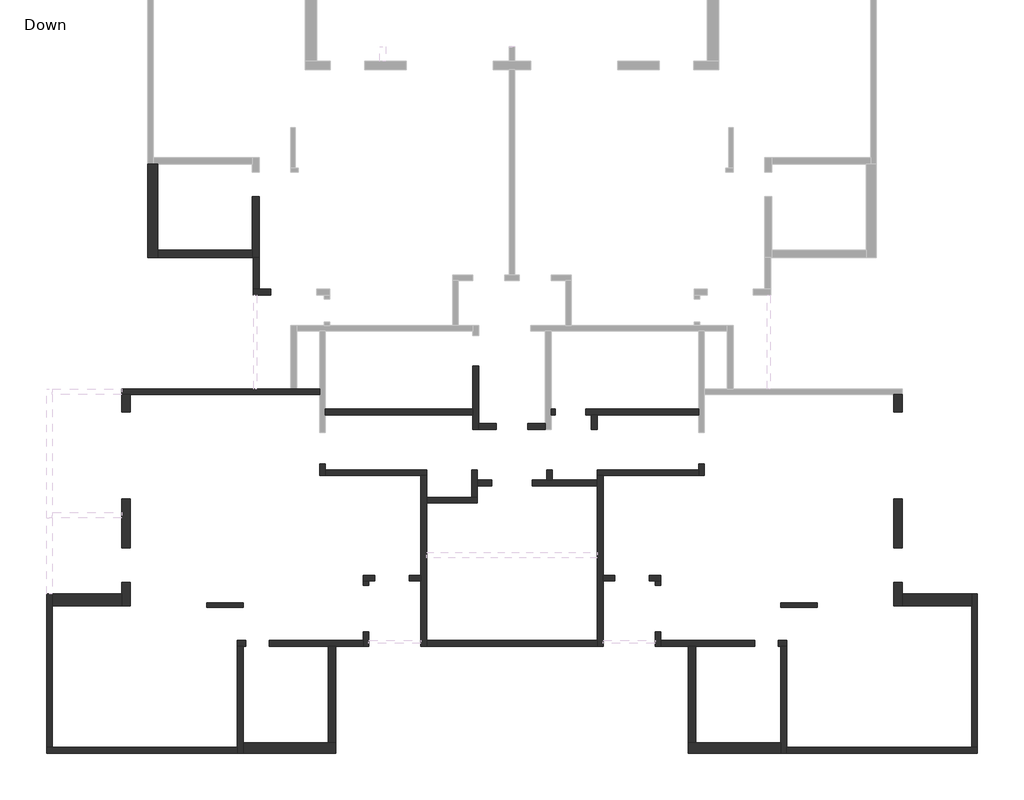
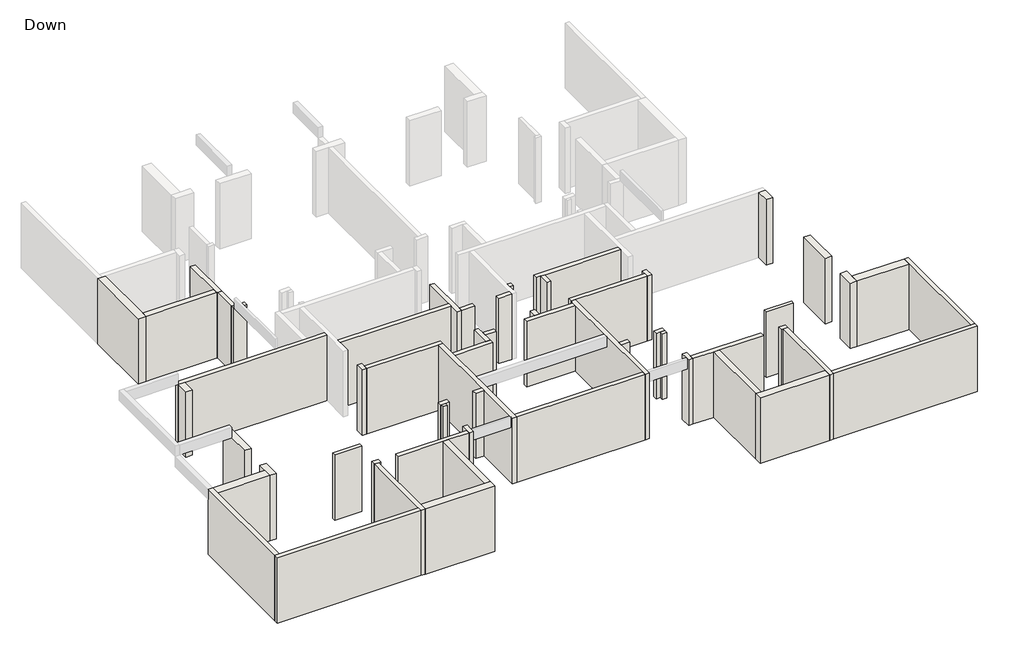
# One storey, part 1 of 2: 57 walls.
"""IFC4 building model written with IfcOpenShell, lengths in millimetres."""

import ifcopenshell
import ifcopenshell.guid

model = None  # the IFC model being written
_history = None  # IfcOwnerHistory: only IFC2X3 demands one
_inside = {}  # id of a spatial element -> (the spatial element, [elements in it])
_under = {}  # id of a project, library or spatial element -> (it, [spatial elements below it])
_declared = {}  # id of a project -> (the project, [libraries it declares])
_typed = {}  # id of a type object -> (the type object, [elements of that type])
_made_of = {}  # id of a material, layer set ... -> (it, [elements and type objects made of it])


def new_model(schema):
    """Start an empty IFC model of exactly this schema.

    Asked for "IFC4X3", IfcOpenShell would pick the latest addendum, in which some entities
    have other attributes; the version numbers below select the first issue.
    IFC2X3 requires an IfcOwnerHistory on every rooted entity: one is made here for all.
    """
    global model, _history
    if schema == "IFC4X3":
        model = ifcopenshell.file(schema_version=(4, 3, 0, 0))
    else:
        model = ifcopenshell.file(schema=schema)
    _inside.clear()
    _under.clear()
    _declared.clear()
    _typed.clear()
    _made_of.clear()
    _history = None
    if model.schema == "IFC2X3":
        org = make("IfcOrganization", Name="unknown")
        user = make(
            "IfcPersonAndOrganization",
            ThePerson=make("IfcPerson", FamilyName="unknown"),
            TheOrganization=org,
        )
        app = make(
            "IfcApplication",
            ApplicationDeveloper=org,
            Version="unknown",
            ApplicationFullName="unknown",
            ApplicationIdentifier="unknown",
        )
        _history = make(
            "IfcOwnerHistory",
            OwningUser=user,
            OwningApplication=app,
            ChangeAction="ADDED",
            CreationDate=0,
        )
    return model


def make(cls, **values):
    """One entity of the class cls with the attributes given. An attribute that is None is left unset."""
    return model.create_entity(
        cls, **{name: value for name, value in values.items() if value is not None}
    )


def rooted(cls, **values):
    """An entity with a GlobalId (a new one), such as an element, a storey or a relation."""
    return make(cls, GlobalId=ifcopenshell.guid.new(), OwnerHistory=_history, **values)


def si_unit(unit_type, name, prefix=None):
    """IfcSIUnit, for example si_unit("LENGTHUNIT", "METRE", prefix="MILLI")."""
    return make("IfcSIUnit", UnitType=unit_type, Prefix=prefix, Name=name)


def assignment(units):
    """IfcUnitAssignment: the units of a project."""
    return None if units is None else make("IfcUnitAssignment", Units=units)


def point(xyz):
    """IfcCartesianPoint."""
    return None if xyz is None else make("IfcCartesianPoint", Coordinates=xyz)


def direction(xyz):
    """IfcDirection."""
    return None if xyz is None else make("IfcDirection", DirectionRatios=xyz)


def frame(location, z_axis=None, x_axis=None):
    """IfcAxis2Placement3D, a coordinate frame: its origin and axes. An axis left out is left unset."""
    return make(
        "IfcAxis2Placement3D",
        Location=point(location),
        Axis=direction(z_axis),
        RefDirection=direction(x_axis),
    )


def origin():
    """The frame at (0, 0, 0) with its axes left unset."""
    return frame((0.0, 0.0, 0.0))


def origin_with_axes():
    """The frame at (0, 0, 0) with the z axis (0, 0, 1) and the x axis (1, 0, 0) written out."""
    return frame((0.0, 0.0, 0.0), z_axis=(0.0, 0.0, 1.0), x_axis=(1.0, 0.0, 0.0))


def place(relative_to, where):
    """IfcLocalPlacement: puts the frame where relative to a parent placement (None: the world)."""
    return make(
        "IfcLocalPlacement", PlacementRelTo=relative_to, RelativePlacement=where
    )


def context(
    kind, dimensions, precision=None, world=None, true_north=None, identifier=None
):
    """IfcGeometricRepresentationContext, for example the 3D "Model" context."""
    return make(
        "IfcGeometricRepresentationContext",
        ContextIdentifier=identifier,
        ContextType=kind,
        CoordinateSpaceDimension=dimensions,
        Precision=precision,
        WorldCoordinateSystem=world,
        TrueNorth=true_north,
    )


def project(units=None, contexts=None):
    """IfcProject with its units and contexts."""
    return rooted(
        "IfcProject",
        Name="project",
        RepresentationContexts=contexts,
        UnitsInContext=assignment(units),
    )


def spatial(cls, under=None, at=None, **own):
    """A site, building, storey or space (cls), placed at a placement, below another one or the project."""
    s = rooted(cls, ObjectPlacement=at, **own)
    if under is not None:
        _under.setdefault(under.id(), (under, []))[1].append(s)
    return s


def polyline(points):
    """IfcPolyline through the points."""
    return make("IfcPolyline", Points=[point(p) for p in points])


def outline(outer, holes=None, kind="AREA"):
    """IfcArbitraryClosedProfileDef: a profile drawn as a closed curve; with holes, ...WithVoids."""
    if holes is None:
        return make("IfcArbitraryClosedProfileDef", ProfileType=kind, OuterCurve=outer)
    return make(
        "IfcArbitraryProfileDefWithVoids",
        ProfileType=kind,
        OuterCurve=outer,
        InnerCurves=holes,
    )


def extrude(swept, where, along, depth):
    """IfcExtrudedAreaSolid: the profile swept, set in the frame where, extruded along a direction by depth."""
    return make(
        "IfcExtrudedAreaSolid",
        SweptArea=swept,
        Position=where,
        ExtrudedDirection=direction(along),
        Depth=depth,
    )


def faces_of(points, faces, orient=None, outer=None):
    """IfcFace entities. A face is a list of loops; a loop is a list of indices into points, from 0.

    orient and outer hold one flag for each loop. By default every Orientation is true, the
    first loop of a face is its IfcFaceOuterBound and the others are IfcFaceBound.
    """
    made = []
    for i, loops in enumerate(faces):
        bounds = []
        for j, loop in enumerate(loops):
            is_outer = j == 0 if outer is None else outer[i][j]
            bounds.append(
                make(
                    "IfcFaceOuterBound" if is_outer else "IfcFaceBound",
                    Bound=make("IfcPolyLoop", Polygon=[points[k] for k in loop]),
                    Orientation=True if orient is None else orient[i][j],
                )
            )
        made.append(make("IfcFace", Bounds=bounds))
    return made


def faceted_brep(points, faces, orient=None, outer=None, voids=None):
    """IfcFacetedBrep: a solid bounded by flat faces; with voids (closed shells), ...WithVoids."""
    shared = [point(p) for p in points]
    hull = make("IfcClosedShell", CfsFaces=faces_of(shared, faces, orient, outer))
    if voids is None:
        return make("IfcFacetedBrep", Outer=hull)
    return make(
        "IfcFacetedBrepWithVoids",
        Outer=hull,
        Voids=[
            make(cls, CfsFaces=faces_of(shared, fs, o, b)) for cls, fs, o, b in voids
        ],
    )


def shape(context_of_items, identifier, shape_type, items):
    """IfcShapeRepresentation: the items that make up one representation, for example the "Body"."""
    return make(
        "IfcShapeRepresentation",
        ContextOfItems=context_of_items,
        RepresentationIdentifier=identifier,
        RepresentationType=shape_type,
        Items=items,
    )


def made_of(thing, what):
    """Note that an element or type object is made of a material, layer set ...; save() writes the relation."""
    if what is not None:
        _made_of.setdefault(what.id(), (what, []))[1].append(thing)
    return thing


def element(
    cls,
    number,
    at=None,
    inside=None,
    cuts=None,
    type_object=None,
    material=None,
    context=None,
    identifier="Body",
    shape_type=None,
    held_by="IfcProductDefinitionShape",
    body=None,
    shapes=None,
    **own,
):
    """One element of the class cls, such as IfcWall. Its Tag is "e" and its number.

    at: its placement. inside: the storey or other place that contains it. cuts: it is an
    opening in that element (IfcRelVoidsElement). A single representation is given by context,
    identifier, shape_type and body (its items); several are given by shapes. held_by: the class
    of the entity that holds the representations. save() writes the other relations.
    """
    e = rooted(cls, Tag="e%d" % number, ObjectPlacement=at, **own)
    if body is not None:
        shapes = [shape(context, identifier, shape_type, body)]
    if shapes is not None:
        e.Representation = make(held_by, Representations=shapes)
    if inside is not None:
        _inside.setdefault(inside.id(), (inside, []))[1].append(e)
    if cuts is not None:
        rooted(
            "IfcRelVoidsElement", RelatingBuildingElement=cuts, RelatedOpeningElement=e
        )
    if type_object is not None:
        _typed.setdefault(type_object.id(), (type_object, []))[1].append(e)
    return made_of(e, material)


def aggregate(whole, parts):
    """IfcRelAggregates: a whole, such as a stair, and the parts it consists of."""
    return rooted("IfcRelAggregates", RelatingObject=whole, RelatedObjects=parts)


def save(model, path):
    """Write the relations noted so far, then the file.

    IfcRelAggregates (storeys below a building ...), IfcRelContainedInSpatialStructure (elements
    in a storey), IfcRelDefinesByType, IfcRelAssociatesMaterial and IfcRelDeclares: one each for
    every whole, place, type object, material and project.
    """
    for whole, parts in _under.values():
        aggregate(whole, parts)
    for where, things in _inside.values():
        rooted(
            "IfcRelContainedInSpatialStructure",
            RelatedElements=things,
            RelatingStructure=where,
        )
    for kind, things in _typed.values():
        rooted("IfcRelDefinesByType", RelatedObjects=things, RelatingType=kind)
    for what, things in _made_of.values():
        rooted("IfcRelAssociatesMaterial", RelatedObjects=things, RelatingMaterial=what)
    for by, libraries in _declared.values():
        rooted("IfcRelDeclares", RelatingContext=by, RelatedDefinitions=libraries)
    model.write(path)


model = new_model("IFC4")

# Units and contexts
model_context = context("Model", 3, world=origin())
ifc_project = project(units=[si_unit("LENGTHUNIT", "METRE", prefix="MILLI")], contexts=[model_context])

# Site, building, storey
site = spatial("IfcSite", under=ifc_project)
building = spatial("IfcBuilding", under=site)
storey = spatial("IfcBuildingStorey", under=building, Name="Down", Elevation=0.0)

# Walls
placement = place(None, origin())
element("IfcWall", 1, ObjectType="15", at=placement, inside=storey, context=model_context, shape_type="Brep", body=[
    faceted_brep([(-10394.9709719, -7272.1211235, 0.0), (-9144.0302381, -7272.1211235, 0.0), (-9144.0302381, -7272.1211235, 2980.0), (-9144.0302381, -7272.1211235, 3180.0), (-10394.9709719, -7272.1211235, 3180.0), (-10394.9709719, -7272.1211235, 2980.0), (-10394.9709719, -7122.1211235, 0.0), (-10394.9709719, -7122.1211235, 2980.0), (-10394.9709719, -7122.1211235, 3180.0), (-9144.0302381, -7122.1211235, 3180.0), (-9144.0302381, -7122.1211235, 2980.0), (-9144.0302381, -7122.1211235, 0.0)], [[[0, 1, 2, 3, 4, 5]], [[6, 7, 8, 9, 10, 11]], [[1, 0, 6, 11]], [[3, 2, 1, 11, 10, 9]], [[4, 3, 9, 8]], [[0, 5, 4, 8, 7, 6]]]),
])
element("IfcWall", 2, ObjectType="15", at=placement, inside=storey, context=model_context, shape_type="Brep", body=[
    faceted_brep([(10709.0741833, -7122.1211235, 0.0), (9458.1334495, -7122.1211235, 0.0), (9458.1334495, -7122.1211235, 2980.0), (9458.1334495, -7122.1211235, 3180.0), (10709.0741833, -7122.1211235, 3180.0), (10709.0741833, -7122.1211235, 2980.0), (10709.0741833, -7272.1211235, 0.0), (10709.0741833, -7272.1211235, 2980.0), (10709.0741833, -7272.1211235, 3180.0), (9458.1334495, -7272.1211235, 3180.0), (9458.1334495, -7272.1211235, 2980.0), (9458.1334495, -7272.1211235, 0.0)], [[[0, 1, 2, 3, 4, 5]], [[6, 7, 8, 9, 10, 11]], [[1, 0, 6, 11]], [[3, 2, 1, 11, 10, 9]], [[4, 3, 9, 8]], [[0, 5, 4, 8, 7, 6]]]),
])
element("IfcWall", 3, ObjectType="20", at=placement, inside=storey, context=model_context, shape_type="Brep", body=[
    faceted_brep([(-8793.7009813, 4828.7725736, 0.0), (-8793.7009813, 3729.1488671, 0.0), (-8793.7009813, 3729.1488671, 3180.0), (-8793.7009813, 4828.7725736, 3180.0), (-8593.7009813, 4828.7725736, 0.0), (-8593.7009813, 4828.7725736, 3180.0), (-8593.7009813, 3729.1488671, 3180.0), (-8593.7009813, 3729.1488671, 2980.0), (-8593.7009813, 3729.1488671, 0.0)], [[[0, 1, 2, 3]], [[4, 5, 6, 7, 8]], [[1, 0, 4, 8]], [[3, 2, 6, 5]], [[0, 3, 5, 4]], [[2, 1, 8, 7, 6]]]),
])
element("IfcWall", 4, ObjectType="20", at=placement, inside=storey, context=model_context, shape_type="Brep", body=[
    faceted_brep([(-8793.7009813, 3529.1488671, 0.0), (-8193.6539446, 3529.1488671, 0.0), (-8193.6539446, 3529.1488671, 2980.0), (-8193.6539446, 3529.1488671, 3180.0), (-8774.1337189, 3529.1488671, 3180.0), (-8793.7009813, 3529.1488671, 3180.0), (-8793.7009813, 3729.1488671, 0.0), (-8793.7009813, 3729.1488671, 3180.0), (-8593.7009813, 3729.1488671, 3180.0), (-8193.6539446, 3729.1488671, 3180.0), (-8193.6539446, 3729.1488671, 2980.0), (-8193.6539446, 3729.1488671, 0.0), (-8593.7009813, 3729.1488671, 0.0)], [[[0, 1, 2, 3, 4, 5]], [[6, 7, 8, 9, 10, 11, 12]], [[1, 0, 6, 12, 11]], [[3, 2, 1, 11, 10, 9]], [[5, 4, 3, 9, 8, 7]], [[0, 5, 7, 6]]]),
])
element("IfcWall", 5, ObjectType="20", at=placement, inside=storey, context=model_context, shape_type="Brep", body=[
    faceted_brep([(-1194.9239352, 1067.4837683, 0.0), (-1194.9239352, -421.6037199, 0.0), (-1194.9239352, -621.6037199, 0.0), (-1194.9239352, -1121.133353, 0.0), (-1194.9239352, -1121.133353, 2980.0), (-1194.9239352, -1121.133353, 3180.0), (-1194.9239352, -621.6037199, 3180.0), (-1194.9239352, -421.6037199, 3180.0), (-1194.9239352, 1067.4837683, 3180.0), (-1194.9239352, 1067.4837683, 2980.0), (-994.9239352, 1067.4837683, 0.0), (-994.9239352, 1067.4837683, 2980.0), (-994.9239352, 1067.4837683, 3180.0), (-994.9239352, -921.133353, 3180.0), (-994.9239352, -1121.133353, 3180.0), (-994.9239352, -1121.133353, 0.0), (-994.9239352, -921.133353, 0.0)], [[[0, 1, 2, 3, 4, 5, 6, 7, 8, 9]], [[10, 11, 12, 13, 14, 15, 16]], [[3, 2, 1, 0, 10, 16, 15]], [[8, 7, 6, 5, 14, 13, 12]], [[0, 9, 8, 12, 11, 10]], [[5, 4, 3, 15, 14]]]),
])
element("IfcWall", 6, ObjectType="20", at=placement, inside=storey, context=model_context, shape_type="Brep", body=[
    faceted_brep([(-994.9239352, -1121.133353, 0.0), (-393.7950547, -1121.133353, 0.0), (-393.7950547, -1121.133353, 2980.0), (-393.7950547, -1121.133353, 3180.0), (-994.9239352, -1121.133353, 3180.0), (-994.9239352, -921.133353, 0.0), (-994.9239352, -921.133353, 2980.0), (-994.9239352, -921.133353, 3180.0), (-393.7950547, -921.133353, 3180.0), (-393.7950547, -921.133353, 2980.0), (-393.7950547, -921.133353, 0.0)], [[[0, 1, 2, 3, 4]], [[5, 6, 7, 8, 9, 10]], [[1, 0, 5, 10]], [[3, 2, 1, 10, 9, 8]], [[4, 3, 8, 7]], [[0, 4, 7, 6, 5]]]),
])
element("IfcWall", 7, ObjectType="20", at=placement, inside=storey, context=model_context, shape_type="Brep", body=[
    faceted_brep([(-1194.9239352, -421.6037199, 0.0), (-6295.0180086, -421.6037199, 0.0), (-6295.0180086, -421.6037199, 3180.0), (-1194.9239352, -421.6037199, 3180.0), (-1194.9239352, -621.6037199, 0.0), (-1194.9239352, -621.6037199, 2980.0), (-1194.9239352, -621.6037199, 3180.0), (-6295.0180086, -621.6037199, 3180.0), (-6295.0180086, -621.6037199, 2980.0), (-6295.0180086, -621.6037199, 0.0)], [[[0, 1, 2, 3]], [[4, 5, 6, 7, 8, 9]], [[1, 0, 4, 9]], [[3, 2, 7, 6]], [[0, 3, 6, 5, 4]], [[2, 1, 9, 8, 7]]]),
])
element("IfcWall", 8, ObjectType="20", at=placement, inside=storey, context=model_context, shape_type="Brep", body=[
    faceted_brep([(-6495.0180086, 279.007757, 0.0), (-7293.0424677, 279.007757, 0.0), (-7493.0424677, 279.007757, 0.0), (-13343.4657979, 279.007757, 0.0), (-13343.4657979, 279.007757, 2980.0), (-13343.4657979, 279.007757, 3180.0), (-8774.1337189, 279.007757, 3180.0), (-7493.0424677, 279.007757, 3180.0), (-7293.0424677, 279.007757, 3180.0), (-6495.0180086, 279.007757, 3180.0), (-6495.0180086, 79.007757, 0.0), (-6495.0180086, 79.007757, 2980.0), (-6495.0180086, 79.007757, 3180.0), (-13042.9013576, 79.007757, 3180.0), (-13342.9013576, 79.007757, 3180.0), (-13343.4657979, 79.007757, 3180.0), (-13343.4657979, 79.007757, 2980.0), (-13343.4657979, 79.007757, 0.0), (-13342.9013576, 79.007757, 0.0), (-13042.9013576, 79.007757, 0.0)], [[[0, 1, 2, 3, 4, 5, 6, 7, 8, 9]], [[10, 11, 12, 13, 14, 15, 16, 17, 18, 19]], [[3, 2, 1, 0, 10, 19, 18, 17]], [[5, 4, 3, 17, 16, 15]], [[9, 8, 7, 6, 5, 15, 14, 13, 12]], [[0, 9, 12, 11, 10]]]),
])
element("IfcWall", 9, ObjectType="20", at=placement, inside=storey, context=model_context, shape_type="Brep", body=[
    faceted_brep([(-6493.9832015, -2321.2744631, 0.0), (-6493.9832015, -2721.3214998, 0.0), (-6493.9832015, -2721.3214998, 2980.0), (-6493.9832015, -2721.3214998, 3180.0), (-6493.9832015, -2321.2744631, 3180.0), (-6493.9832015, -2321.2744631, 2980.0), (-6293.9832015, -2321.2744631, 0.0), (-6293.9832015, -2321.2744631, 2980.0), (-6293.9832015, -2321.2744631, 3180.0), (-6293.9832015, -2521.3214998, 3180.0), (-6293.9832015, -2721.3214998, 3180.0), (-6293.9832015, -2721.3214998, 0.0), (-6293.9832015, -2521.3214998, 0.0), (-6295.0180086, -2321.2744631, 3180.0)], [[[0, 1, 2, 3, 4, 5]], [[6, 7, 8, 9, 10, 11, 12]], [[1, 0, 6, 12, 11]], [[4, 3, 10, 9, 8, 13]], [[0, 5, 4, 13, 8, 7, 6]], [[3, 2, 1, 11, 10]]]),
])
element("IfcWall", 10, ObjectType="20", at=placement, inside=storey, context=model_context, shape_type="Brep", body=[
    faceted_brep([(-6293.9832015, -2721.3214998, 0.0), (-2993.9832015, -2721.3214998, 0.0), (-2793.9832015, -2721.3214998, 0.0), (-2793.9832015, -2721.3214998, 3180.0), (-2993.9832015, -2721.3214998, 3180.0), (-6293.9832015, -2721.3214998, 3180.0), (-6293.9832015, -2521.3214998, 0.0), (-6293.9832015, -2521.3214998, 2980.0), (-6293.9832015, -2521.3214998, 3180.0), (-2793.9832015, -2521.3214998, 3180.0), (-2793.9832015, -2521.3214998, 2980.0), (-2793.9832015, -2521.3214998, 0.0)], [[[0, 1, 2, 3, 4, 5]], [[6, 7, 8, 9, 10, 11]], [[2, 1, 0, 6, 11]], [[5, 4, 3, 9, 8]], [[0, 5, 8, 7, 6]], [[3, 2, 11, 10, 9]]]),
])
element("IfcWall", 11, ObjectType="20", at=placement, inside=storey, context=model_context, shape_type="Brep", body=[
    faceted_brep([(-2993.9832015, -2721.3214998, 0.0), (-2993.9832015, -6171.4626098, 0.0), (-2993.9832015, -6371.4626098, 0.0), (-2993.9832015, -8622.5444537, 0.0), (-2993.9832015, -8622.5444537, 3180.0), (-2993.9832015, -8420.9452063, 3180.0), (-2993.9832015, -6371.4626098, 3180.0), (-2993.9832015, -6171.4626098, 3180.0), (-2993.9832015, -2721.3214998, 3180.0), (-2993.9832015, -2721.3214998, 2980.0), (-2793.9832015, -2721.3214998, 0.0), (-2793.9832015, -2721.3214998, 3180.0), (-2793.9832015, -3471.6977933, 3180.0), (-2793.9832015, -3671.6977933, 3180.0), (-2793.9832015, -5372.4503803, 3180.0), (-2793.9832015, -8422.5444537, 3180.0), (-2793.9832015, -8622.5444537, 3180.0), (-2793.9832015, -8622.5444537, 0.0), (-2793.9832015, -8422.5444537, 0.0), (-2793.9832015, -3671.6977933, 0.0), (-2793.9832015, -3471.6977933, 0.0)], [[[0, 1, 2, 3, 4, 5, 6, 7, 8, 9]], [[10, 11, 12, 13, 14, 15, 16, 17, 18, 19, 20]], [[3, 2, 1, 0, 10, 20, 19, 18, 17]], [[8, 7, 6, 5, 4, 16, 15, 14, 13, 12, 11]], [[0, 9, 8, 11, 10]], [[4, 3, 17, 16]]]),
])
element("IfcWall", 12, ObjectType="20", at=placement, inside=storey, context=model_context, shape_type="Brep", body=[
    faceted_brep([(-2993.9832015, -6171.4626098, 0.0), (-3395.2061554, -6171.4626098, 0.0), (-3395.2061554, -6171.4626098, 2980.0), (-3395.2061554, -6171.4626098, 3180.0), (-2993.9832015, -6171.4626098, 3180.0), (-2993.9832015, -6171.4626098, 2980.0), (-2993.9832015, -6371.4626098, 0.0), (-2993.9832015, -6371.4626098, 2980.0), (-2993.9832015, -6371.4626098, 3180.0), (-3395.2061554, -6371.4626098, 3180.0), (-3395.2061554, -6371.4626098, 2980.0), (-3395.2061554, -6371.4626098, 0.0)], [[[0, 1, 2, 3, 4, 5]], [[6, 7, 8, 9, 10, 11]], [[1, 0, 6, 11]], [[3, 2, 1, 11, 10, 9]], [[4, 3, 9, 8]], [[0, 5, 4, 8, 7, 6]]]),
])
element("IfcWall", 13, ObjectType="20", at=placement, inside=storey, context=model_context, shape_type="Brep", body=[
    faceted_brep([(-4595.3472654, -6171.4626098, 0.0), (-4993.2776511, -6171.4626098, 0.0), (-4993.2776511, -6171.4626098, 2980.0), (-4993.2776511, -6171.4626098, 3180.0), (-4595.3472654, -6171.4626098, 3180.0), (-4595.3472654, -6171.4626098, 2980.0), (-4595.3472654, -6371.4626098, 0.0), (-4595.3472654, -6371.4626098, 2980.0), (-4595.3472654, -6371.4626098, 3180.0), (-4793.2776511, -6371.4626098, 3180.0), (-4993.2776511, -6371.4626098, 3180.0), (-4993.2776511, -6371.4626098, 0.0), (-4793.2776511, -6371.4626098, 0.0)], [[[0, 1, 2, 3, 4, 5]], [[6, 7, 8, 9, 10, 11, 12]], [[1, 0, 6, 12, 11]], [[4, 3, 10, 9, 8]], [[0, 5, 4, 8, 7, 6]], [[3, 2, 1, 11, 10]]]),
])
element("IfcWall", 14, ObjectType="20", at=placement, inside=storey, context=model_context, shape_type="Brep", body=[
    faceted_brep([(-4993.2776511, -6371.4626098, 0.0), (-4993.2776511, -6522.8266738, 0.0), (-4993.2776511, -6522.8266738, 2980.0), (-4993.2776511, -6522.8266738, 3180.0), (-4993.2776511, -6371.4626098, 3180.0), (-4793.2776511, -6371.4626098, 0.0), (-4793.2776511, -6371.4626098, 2980.0), (-4793.2776511, -6371.4626098, 3180.0), (-4793.2776511, -6522.8266738, 3180.0), (-4793.2776511, -6522.8266738, 2980.0), (-4793.2776511, -6522.8266738, 0.0)], [[[0, 1, 2, 3, 4]], [[5, 6, 7, 8, 9, 10]], [[1, 0, 5, 10]], [[3, 2, 1, 10, 9, 8]], [[4, 3, 8, 7]], [[0, 4, 7, 6, 5]]]),
])
element("IfcWall", 15, ObjectType="20", at=placement, inside=storey, context=model_context, shape_type="Brep", body=[
    faceted_brep([(-4993.2776511, -8120.8981696, 0.0), (-4993.2776511, -8422.5444537, 0.0), (-4993.2776511, -8622.5444537, 0.0), (-4993.2776511, -8622.5444537, 3180.0), (-4993.2776511, -8422.5444537, 3180.0), (-4993.2776511, -8120.8981696, 3180.0), (-4993.2776511, -8120.8981696, 2980.0), (-4793.2776511, -8120.8981696, 0.0), (-4793.2776511, -8120.8981696, 2980.0), (-4793.2776511, -8120.8981696, 3180.0), (-4793.2776511, -8420.9452063, 3180.0), (-4793.2776511, -8622.5444537, 3180.0), (-4793.2776511, -8622.5444537, 0.0)], [[[0, 1, 2, 3, 4, 5, 6]], [[7, 8, 9, 10, 11, 12]], [[2, 1, 0, 7, 12]], [[5, 4, 3, 11, 10, 9]], [[0, 6, 5, 9, 8, 7]], [[3, 2, 12, 11]]]),
])
element("IfcWall", 16, ObjectType="20", at=placement, inside=storey, context=model_context, shape_type="Brep", body=[
    faceted_brep([(-4993.2776511, -8422.5444537, 0.0), (-8238.1036154, -8422.5444537, 0.0), (-8238.1036154, -8422.5444537, 2980.0), (-8238.1036154, -8422.5444537, 3180.0), (-4993.2776511, -8422.5444537, 3180.0), (-4993.2776511, -8422.5444537, 2980.0), (-4993.2776511, -8622.5444537, 0.0), (-4993.2776511, -8622.5444537, 3180.0), (-5943.7809437, -8622.5444537, 3180.0), (-6193.7809437, -8622.5444537, 3180.0), (-8238.1036154, -8622.5444537, 3180.0), (-8238.1036154, -8622.5444537, 2980.0), (-8238.1036154, -8622.5444537, 0.0), (-6193.7809437, -8622.5444537, 0.0), (-5943.7809437, -8622.5444537, 0.0)], [[[0, 1, 2, 3, 4, 5]], [[6, 7, 8, 9, 10, 11, 12, 13, 14]], [[1, 0, 6, 14, 13, 12]], [[3, 2, 1, 12, 11, 10]], [[4, 3, 10, 9, 8, 7]], [[0, 5, 4, 7, 6]]]),
])
element("IfcWall", 17, ObjectType="20", at=placement, inside=storey, context=model_context, shape_type="Brep", body=[
    faceted_brep([(-9048.7809437, -8422.5444537, 0.0), (-9343.7809437, -8422.5444537, 0.0), (-9343.7809437, -8422.5444537, 2980.0), (-9343.7809437, -8422.5444537, 3180.0), (-9048.7809437, -8422.5444537, 3180.0), (-9048.7809437, -8422.5444537, 2980.0), (-9048.7809437, -8622.5444537, 0.0), (-9048.7809437, -8622.5444537, 2980.0), (-9048.7809437, -8622.5444537, 3180.0), (-9143.7809437, -8622.5444537, 3180.0), (-9343.7809437, -8622.5444537, 3180.0), (-9343.7809437, -8622.5444537, 0.0), (-9143.7809437, -8622.5444537, 0.0)], [[[0, 1, 2, 3, 4, 5]], [[6, 7, 8, 9, 10, 11, 12]], [[1, 0, 6, 12, 11]], [[4, 3, 10, 9, 8]], [[0, 5, 4, 8, 7, 6]], [[3, 2, 1, 11, 10]]]),
])
element("IfcWall", 18, ObjectType="20", at=placement, inside=storey, context=model_context, shape_type="Brep", body=[
    faceted_brep([(-9343.7809437, -8622.5444537, 0.0), (-9343.7809437, -12122.4503803, 0.0), (-9343.7809437, -12322.4503803, 0.0), (-9343.7809437, -12322.4503803, 3180.0), (-9343.7809437, -12122.4503803, 3180.0), (-9343.7809437, -8622.5444537, 3180.0), (-9143.7809437, -8622.5444537, 0.0), (-9143.7809437, -8622.5444537, 2980.0), (-9143.7809437, -8622.5444537, 3180.0), (-9143.7809437, -11972.4503803, 3180.0), (-9143.7809437, -12322.4503803, 3180.0), (-9143.7809437, -12322.4503803, 0.0), (-9143.7809437, -11972.4503803, 0.0)], [[[0, 1, 2, 3, 4, 5]], [[6, 7, 8, 9, 10, 11, 12]], [[2, 1, 0, 6, 12, 11]], [[5, 4, 3, 10, 9, 8]], [[0, 5, 8, 7, 6]], [[3, 2, 11, 10]]]),
])
element("IfcWall", 19, ObjectType="20", at=placement, inside=storey, context=model_context, shape_type="Brep", body=[
    faceted_brep([(-9343.7809437, -12122.4503803, 0.0), (-15742.7132109, -12122.4503803, 0.0), (-15942.7132109, -12122.4503803, 0.0), (-15942.7132109, -12122.4503803, 3180.0), (-15742.7132109, -12122.4503803, 3180.0), (-9343.7809437, -12122.4503803, 3180.0), (-9343.7809437, -12122.4503803, 2980.0), (-9343.7809437, -12322.4503803, 0.0), (-9343.7809437, -12322.4503803, 3180.0), (-15942.7132109, -12322.4503803, 3180.0), (-15942.7132109, -12322.4503803, 0.0)], [[[0, 1, 2, 3, 4, 5, 6]], [[7, 8, 9, 10]], [[2, 1, 0, 7, 10]], [[5, 4, 3, 9, 8]], [[3, 2, 10, 9]], [[0, 6, 5, 8, 7]]]),
])
element("IfcWall", 20, ObjectType="20", at=placement, inside=storey, context=model_context, shape_type="Brep", body=[
    faceted_brep([(-15742.7132109, -12122.4503803, 0.0), (-15742.7132109, -7221.2744631, 0.0), (-15742.7132109, -6821.2744631, 0.0), (-15742.7132109, -6821.2744631, 2680.0), (-15742.7132109, -6821.2744631, 3180.0), (-15742.7132109, -7221.2744631, 3180.0), (-15742.7132109, -12122.4503803, 3180.0), (-15742.7132109, -12122.4503803, 2980.0), (-15942.7132109, -12122.4503803, 0.0), (-15942.7132109, -12122.4503803, 3180.0), (-15942.7132109, -6821.2744631, 3180.0), (-15942.7132109, -6821.2744631, 2680.0), (-15942.7132109, -6821.2744631, 0.0)], [[[0, 1, 2, 3, 4, 5, 6, 7]], [[8, 9, 10, 11, 12]], [[2, 1, 0, 8, 12]], [[6, 5, 4, 10, 9]], [[0, 7, 6, 9, 8]], [[4, 3, 2, 12, 11, 10]]]),
])
element("IfcWall", 21, ObjectType="20", at=placement, inside=storey, context=model_context, shape_type="Brep", body=[
    faceted_brep([(1309.0271466, -921.133353, 0.0), (707.8982661, -921.133353, 0.0), (707.8982661, -921.133353, 2980.0), (707.8982661, -921.133353, 3180.0), (1309.0271466, -921.133353, 3180.0), (1309.0271466, -921.133353, 2980.0), (1309.0271466, -1121.133353, 0.0), (1309.0271466, -1121.133353, 3180.0), (707.8982661, -1121.133353, 3180.0), (707.8982661, -1121.133353, 2980.0), (707.8982661, -1121.133353, 0.0)], [[[0, 1, 2, 3, 4, 5]], [[6, 7, 8, 9, 10]], [[1, 0, 6, 10]], [[3, 2, 1, 10, 9, 8]], [[4, 3, 8, 7]], [[0, 5, 4, 7, 6]]]),
])
element("IfcWall", 22, ObjectType="20", at=placement, inside=storey, context=model_context, shape_type="Brep", body=[
    faceted_brep([(2709.12122, -621.6037199, 0.0), (2906.0638352, -621.6037199, 0.0), (3106.0638352, -621.6037199, 0.0), (6609.12122, -621.6037199, 0.0), (6609.12122, -621.6037199, 2980.0), (6609.12122, -621.6037199, 3180.0), (3106.0638352, -621.6037199, 3180.0), (2906.0638352, -621.6037199, 3180.0), (2709.12122, -621.6037199, 3180.0), (2709.12122, -621.6037199, 2980.0), (2709.12122, -421.6037199, 0.0), (2709.12122, -421.6037199, 2980.0), (2709.12122, -421.6037199, 3180.0), (6609.12122, -421.6037199, 3180.0), (6609.12122, -421.6037199, 0.0)], [[[0, 1, 2, 3, 4, 5, 6, 7, 8, 9]], [[10, 11, 12, 13, 14]], [[3, 2, 1, 0, 10, 14]], [[8, 7, 6, 5, 13, 12]], [[0, 9, 8, 12, 11, 10]], [[5, 4, 3, 14, 13]]]),
])
element("IfcWall", 23, ObjectType="20", at=placement, inside=storey, context=model_context, shape_type="Brep", body=[
    faceted_brep([(6608.0864128, -2321.2744631, 0.0), (6608.0864128, -2521.3214998, 0.0), (6608.0864128, -2721.3214998, 0.0), (6608.0864128, -2721.3214998, 3180.0), (6608.0864128, -2521.3214998, 3180.0), (6608.0864128, -2321.2744631, 3180.0), (6608.0864128, -2321.2744631, 2980.0), (6808.0864128, -2321.2744631, 0.0), (6808.0864128, -2321.2744631, 2980.0), (6808.0864128, -2321.2744631, 3180.0), (6808.0864128, -2721.3214998, 3180.0), (6808.0864128, -2721.3214998, 2980.0), (6808.0864128, -2721.3214998, 0.0), (6609.12122, -2321.2744631, 3180.0)], [[[0, 1, 2, 3, 4, 5, 6]], [[7, 8, 9, 10, 11, 12]], [[2, 1, 0, 7, 12]], [[5, 4, 3, 10, 9, 13]], [[0, 6, 5, 13, 9, 8, 7]], [[3, 2, 12, 11, 10]]]),
])
element("IfcWall", 24, ObjectType="20", at=placement, inside=storey, context=model_context, shape_type="Brep", body=[
    faceted_brep([(6608.0864128, -2521.3214998, 0.0), (3108.0864128, -2521.3214998, 0.0), (3108.0864128, -2521.3214998, 2980.0), (3108.0864128, -2521.3214998, 3180.0), (6608.0864128, -2521.3214998, 3180.0), (6608.0864128, -2521.3214998, 2980.0), (6608.0864128, -2721.3214998, 0.0), (6608.0864128, -2721.3214998, 3180.0), (3308.0864128, -2721.3214998, 3180.0), (3108.0864128, -2721.3214998, 3180.0), (3108.0864128, -2721.3214998, 0.0), (3308.0864128, -2721.3214998, 0.0)], [[[0, 1, 2, 3, 4, 5]], [[6, 7, 8, 9, 10, 11]], [[1, 0, 6, 11, 10]], [[4, 3, 9, 8, 7]], [[0, 5, 4, 7, 6]], [[3, 2, 1, 10, 9]]]),
])
element("IfcWall", 25, ObjectType="20", at=placement, inside=storey, context=model_context, shape_type="Brep", body=[
    faceted_brep([(3108.0864128, -2721.3214998, 0.0), (3108.0864128, -2872.6855637, 0.0), (3108.0864128, -3072.6855637, 0.0), (3108.0864128, -8422.5444537, 0.0), (3108.0864128, -8622.5444537, 0.0), (3108.0864128, -8622.5444537, 3180.0), (3108.0864128, -8422.5444537, 3180.0), (3108.0864128, -5372.4503803, 3180.0), (3108.0864128, -3072.6855637, 3180.0), (3108.0864128, -2872.6855637, 3180.0), (3108.0864128, -2721.3214998, 3180.0), (3308.0864128, -2721.3214998, 0.0), (3308.0864128, -2721.3214998, 2980.0), (3308.0864128, -2721.3214998, 3180.0), (3308.0864128, -6171.4626098, 3180.0), (3308.0864128, -6371.4626098, 3180.0), (3308.0864128, -8420.9495778, 3180.0), (3308.0864128, -8622.5444537, 3180.0), (3308.0864128, -8622.5444537, 0.0), (3308.0864128, -6371.4626098, 0.0), (3308.0864128, -6171.4626098, 0.0)], [[[0, 1, 2, 3, 4, 5, 6, 7, 8, 9, 10]], [[11, 12, 13, 14, 15, 16, 17, 18, 19, 20]], [[4, 3, 2, 1, 0, 11, 20, 19, 18]], [[10, 9, 8, 7, 6, 5, 17, 16, 15, 14, 13]], [[0, 10, 13, 12, 11]], [[5, 4, 18, 17]]]),
])
element("IfcWall", 26, ObjectType="20", at=placement, inside=storey, context=model_context, shape_type="Brep", body=[
    faceted_brep([(3308.0864128, -6371.4626098, 0.0), (3709.3093668, -6371.4626098, 0.0), (3709.3093668, -6371.4626098, 2980.0), (3709.3093668, -6371.4626098, 3180.0), (3308.0864128, -6371.4626098, 3180.0), (3308.0864128, -6371.4626098, 2980.0), (3308.0864128, -6171.4626098, 0.0), (3308.0864128, -6171.4626098, 2980.0), (3308.0864128, -6171.4626098, 3180.0), (3709.3093668, -6171.4626098, 3180.0), (3709.3093668, -6171.4626098, 2980.0), (3709.3093668, -6171.4626098, 0.0)], [[[0, 1, 2, 3, 4, 5]], [[6, 7, 8, 9, 10, 11]], [[1, 0, 6, 11]], [[3, 2, 1, 11, 10, 9]], [[4, 3, 9, 8]], [[0, 5, 4, 8, 7, 6]]]),
])
element("IfcWall", 27, ObjectType="20", at=placement, inside=storey, context=model_context, shape_type="Brep", body=[
    faceted_brep([(4909.4504768, -6371.4626098, 0.0), (5107.3808625, -6371.4626098, 0.0), (5307.3808625, -6371.4626098, 0.0), (5307.3808625, -6371.4626098, 3180.0), (5107.3808625, -6371.4626098, 3180.0), (4909.4504768, -6371.4626098, 3180.0), (4909.4504768, -6371.4626098, 2980.0), (4909.4504768, -6171.4626098, 0.0), (4909.4504768, -6171.4626098, 2980.0), (4909.4504768, -6171.4626098, 3180.0), (5307.3808625, -6171.4626098, 3180.0), (5307.3808625, -6171.4626098, 2980.0), (5307.3808625, -6171.4626098, 0.0)], [[[0, 1, 2, 3, 4, 5, 6]], [[7, 8, 9, 10, 11, 12]], [[2, 1, 0, 7, 12]], [[5, 4, 3, 10, 9]], [[0, 6, 5, 9, 8, 7]], [[3, 2, 12, 11, 10]]]),
])
element("IfcWall", 28, ObjectType="20", at=placement, inside=storey, context=model_context, shape_type="Brep", body=[
    faceted_brep([(5107.3808625, -6371.4626098, 0.0), (5107.3808625, -6522.8266738, 0.0), (5107.3808625, -6522.8266738, 2980.0), (5107.3808625, -6522.8266738, 3180.0), (5107.3808625, -6371.4626098, 3180.0), (5107.3808625, -6371.4626098, 2980.0), (5307.3808625, -6371.4626098, 0.0), (5307.3808625, -6371.4626098, 3180.0), (5307.3808625, -6522.8266738, 3180.0), (5307.3808625, -6522.8266738, 2980.0), (5307.3808625, -6522.8266738, 0.0)], [[[0, 1, 2, 3, 4, 5]], [[6, 7, 8, 9, 10]], [[1, 0, 6, 10]], [[3, 2, 1, 10, 9, 8]], [[4, 3, 8, 7]], [[0, 5, 4, 7, 6]]]),
])
element("IfcWall", 29, ObjectType="20", at=placement, inside=storey, context=model_context, shape_type="Brep", body=[
    faceted_brep([(5107.3808625, -8120.8981696, 0.0), (5107.3808625, -8622.5444537, 0.0), (5107.3808625, -8622.5444537, 3180.0), (5107.3808625, -8420.9495778, 3180.0), (5107.3808625, -8120.8981696, 3180.0), (5107.3808625, -8120.8981696, 2980.0), (5307.3808625, -8120.8981696, 0.0), (5307.3808625, -8120.8981696, 2980.0), (5307.3808625, -8120.8981696, 3180.0), (5307.3808625, -8422.5444537, 3180.0), (5307.3808625, -8622.5444537, 3180.0), (5307.3808625, -8622.5444537, 0.0), (5307.3808625, -8422.5444537, 0.0)], [[[0, 1, 2, 3, 4, 5]], [[6, 7, 8, 9, 10, 11, 12]], [[1, 0, 6, 12, 11]], [[4, 3, 2, 10, 9, 8]], [[0, 5, 4, 8, 7, 6]], [[2, 1, 11, 10]]]),
])
element("IfcWall", 30, ObjectType="20", at=placement, inside=storey, context=model_context, shape_type="Brep", body=[
    faceted_brep([(5307.3808625, -8622.5444537, 0.0), (6257.8841551, -8622.5444537, 0.0), (6507.8841551, -8622.5444537, 0.0), (8552.2068268, -8622.5444537, 0.0), (8552.2068268, -8622.5444537, 2980.0), (8552.2068268, -8622.5444537, 3180.0), (6507.8841551, -8622.5444537, 3180.0), (6257.8841551, -8622.5444537, 3180.0), (5307.3808625, -8622.5444537, 3180.0), (5307.3808625, -8422.5444537, 0.0), (5307.3808625, -8422.5444537, 2980.0), (5307.3808625, -8422.5444537, 3180.0), (8552.2068268, -8422.5444537, 3180.0), (8552.2068268, -8422.5444537, 2980.0), (8552.2068268, -8422.5444537, 0.0)], [[[0, 1, 2, 3, 4, 5, 6, 7, 8]], [[9, 10, 11, 12, 13, 14]], [[3, 2, 1, 0, 9, 14]], [[5, 4, 3, 14, 13, 12]], [[8, 7, 6, 5, 12, 11]], [[0, 8, 11, 10, 9]]]),
])
element("IfcWall", 31, ObjectType="20", at=placement, inside=storey, context=model_context, shape_type="Brep", body=[
    faceted_brep([(9362.8841551, -8622.5444537, 0.0), (9457.8841551, -8622.5444537, 0.0), (9657.8841551, -8622.5444537, 0.0), (9657.8841551, -8622.5444537, 3180.0), (9457.8841551, -8622.5444537, 3180.0), (9362.8841551, -8622.5444537, 3180.0), (9362.8841551, -8622.5444537, 2980.0), (9362.8841551, -8422.5444537, 0.0), (9362.8841551, -8422.5444537, 2980.0), (9362.8841551, -8422.5444537, 3180.0), (9657.8841551, -8422.5444537, 3180.0), (9657.8841551, -8422.5444537, 2980.0), (9657.8841551, -8422.5444537, 0.0)], [[[0, 1, 2, 3, 4, 5, 6]], [[7, 8, 9, 10, 11, 12]], [[2, 1, 0, 7, 12]], [[5, 4, 3, 10, 9]], [[0, 6, 5, 9, 8, 7]], [[3, 2, 12, 11, 10]]]),
])
element("IfcWall", 32, ObjectType="20", at=placement, inside=storey, context=model_context, shape_type="Brep", body=[
    faceted_brep([(9457.8841551, -8622.5444537, 0.0), (9457.8841551, -11972.4503803, 0.0), (9457.8841551, -12322.4503803, 0.0), (9457.8841551, -12322.4503803, 3180.0), (9457.8841551, -11972.4503803, 3180.0), (9457.8841551, -8622.5444537, 3180.0), (9457.8841551, -8622.5444537, 2980.0), (9657.8841551, -8622.5444537, 0.0), (9657.8841551, -8622.5444537, 3180.0), (9657.8841551, -12122.4503803, 3180.0), (9657.8841551, -12322.4503803, 3180.0), (9657.8841551, -12322.4503803, 0.0), (9657.8841551, -12122.4503803, 0.0)], [[[0, 1, 2, 3, 4, 5, 6]], [[7, 8, 9, 10, 11, 12]], [[2, 1, 0, 7, 12, 11]], [[5, 4, 3, 10, 9, 8]], [[0, 6, 5, 8, 7]], [[3, 2, 11, 10]]]),
])
element("IfcWall", 33, ObjectType="20", at=placement, inside=storey, context=model_context, shape_type="Brep", body=[
    faceted_brep([(9657.8841551, -12322.4503803, 0.0), (16256.8164223, -12322.4503803, 0.0), (16256.8164223, -12322.4503803, 3180.0), (9657.8841551, -12322.4503803, 3180.0), (9657.8841551, -12122.4503803, 0.0), (9657.8841551, -12122.4503803, 2980.0), (9657.8841551, -12122.4503803, 3180.0), (16056.8164223, -12122.4503803, 3180.0), (16256.8164223, -12122.4503803, 3180.0), (16256.8164223, -12122.4503803, 0.0), (16056.8164223, -12122.4503803, 0.0)], [[[0, 1, 2, 3]], [[4, 5, 6, 7, 8, 9, 10]], [[1, 0, 4, 10, 9]], [[3, 2, 8, 7, 6]], [[2, 1, 9, 8]], [[0, 3, 6, 5, 4]]]),
])
element("IfcWall", 34, ObjectType="20", at=placement, inside=storey, context=model_context, shape_type="Brep", body=[
    faceted_brep([(16256.8164223, -12122.4503803, 0.0), (16256.8164223, -6821.2744631, 0.0), (16256.8164223, -6821.2744631, 2680.0), (16256.8164223, -6821.2744631, 3180.0), (16256.8164223, -12122.4503803, 3180.0), (16056.8164223, -12122.4503803, 0.0), (16056.8164223, -12122.4503803, 2980.0), (16056.8164223, -12122.4503803, 3180.0), (16056.8164223, -7221.2744631, 3180.0), (16056.8164223, -6821.2744631, 3180.0), (16056.8164223, -6821.2744631, 2680.0), (16056.8164223, -6821.2744631, 0.0), (16056.8164223, -7221.2744631, 0.0)], [[[0, 1, 2, 3, 4]], [[5, 6, 7, 8, 9, 10, 11, 12]], [[1, 0, 5, 12, 11]], [[4, 3, 9, 8, 7]], [[0, 4, 7, 6, 5]], [[3, 2, 1, 11, 10, 9]]]),
])
element("IfcWall", 35, ObjectType="20", at=placement, inside=storey, context=model_context, shape_type="Brep", body=[
    faceted_brep([(3106.0638352, -1121.133353, 0.0), (3106.0638352, -621.6037199, 0.0), (3106.0638352, -621.6037199, 2980.0), (3106.0638352, -621.6037199, 3180.0), (3106.0638352, -1121.133353, 3180.0), (3106.0638352, -1121.133353, 2980.0), (2906.0638352, -1121.133353, 0.0), (2906.0638352, -1121.133353, 2980.0), (2906.0638352, -1121.133353, 3180.0), (2906.0638352, -621.6037199, 3180.0), (2906.0638352, -621.6037199, 2980.0), (2906.0638352, -621.6037199, 0.0)], [[[0, 1, 2, 3, 4, 5]], [[6, 7, 8, 9, 10, 11]], [[1, 0, 6, 11]], [[4, 3, 9, 8]], [[0, 5, 4, 8, 7, 6]], [[3, 2, 1, 11, 10, 9]]]),
])
element("IfcWall", 36, ObjectType="20", at=placement, inside=storey, context=model_context, shape_type="Brep", body=[
    faceted_brep([(1509.0271466, -622.6385271, 0.0), (1655.1231015, -622.6385271, 0.0), (1655.1231015, -622.6385271, 2980.0), (1655.1231015, -622.6385271, 3180.0), (1509.0271466, -622.6385271, 3180.0), (1509.0271466, -622.6385271, 2980.0), (1509.0271466, -422.6385271, 0.0), (1509.0271466, -422.6385271, 3180.0), (1655.1231015, -422.6385271, 3180.0), (1655.1231015, -422.6385271, 0.0)], [[[0, 1, 2, 3, 4, 5]], [[6, 7, 8, 9]], [[1, 0, 6, 9]], [[3, 2, 1, 9, 8]], [[4, 3, 8, 7]], [[0, 5, 4, 7, 6]]]),
])
element("IfcWall", 37, ObjectType="20", at=placement, inside=storey, context=model_context, shape_type="SweptSolid", body=[
    extrude(outline(polyline([(3108.0864128, -8622.5444537), (-2793.9832015, -8622.5444537), (-2793.9832015, -8422.5444537), (3108.0864128, -8422.5444537), (3108.0864128, -8622.5444537)])), origin_with_axes(), (0.0, 0.0, 1.0), 3180.0),
])
element("IfcWall", 38, ObjectType="20", at=placement, inside=storey, context=model_context, shape_type="Brep", body=[
    faceted_brep([(-2793.9832015, -3671.6977933, 0.0), (-1043.6069079, -3671.6977933, 0.0), (-1043.6069079, -3671.6977933, 2980.0), (-1043.6069079, -3671.6977933, 3180.0), (-2793.9832015, -3671.6977933, 3180.0), (-2793.9832015, -3671.6977933, 2980.0), (-2793.9832015, -3471.6977933, 0.0), (-2793.9832015, -3471.6977933, 2980.0), (-2793.9832015, -3471.6977933, 3180.0), (-1243.6069079, -3471.6977933, 3180.0), (-1043.6069079, -3471.6977933, 3180.0), (-1043.6069079, -3471.6977933, 0.0), (-1243.6069079, -3471.6977933, 0.0)], [[[0, 1, 2, 3, 4, 5]], [[6, 7, 8, 9, 10, 11, 12]], [[1, 0, 6, 12, 11]], [[4, 3, 10, 9, 8]], [[0, 5, 4, 8, 7, 6]], [[3, 2, 1, 11, 10]]]),
])
element("IfcWall", 39, ObjectType="20", at=placement, inside=storey, context=model_context, shape_type="Brep", body=[
    faceted_brep([(-1043.6069079, -3471.6977933, 0.0), (-1043.6069079, -3071.6037199, 0.0), (-1043.6069079, -2871.6037199, 0.0), (-1043.6069079, -2526.6037199, 0.0), (-1043.6069079, -2526.6037199, 2980.0), (-1043.6069079, -2526.6037199, 3180.0), (-1043.6069079, -2871.6037199, 3180.0), (-1043.6069079, -3071.6037199, 3180.0), (-1043.6069079, -3471.6977933, 3180.0), (-1243.6069079, -3471.6977933, 0.0), (-1243.6069079, -3471.6977933, 2980.0), (-1243.6069079, -3471.6977933, 3180.0), (-1243.6069079, -2526.6037199, 3180.0), (-1243.6069079, -2526.6037199, 2980.0), (-1243.6069079, -2526.6037199, 0.0)], [[[0, 1, 2, 3, 4, 5, 6, 7, 8]], [[9, 10, 11, 12, 13, 14]], [[3, 2, 1, 0, 9, 14]], [[5, 4, 3, 14, 13, 12]], [[8, 7, 6, 5, 12, 11]], [[0, 8, 11, 10, 9]]]),
])
element("IfcWall", 40, ObjectType="20", at=placement, inside=storey, context=model_context, shape_type="Brep", body=[
    faceted_brep([(-1043.6069079, -3071.6037199, 0.0), (-544.0772748, -3071.6037199, 0.0), (-544.0772748, -3071.6037199, 2980.0), (-544.0772748, -3071.6037199, 3180.0), (-1043.6069079, -3071.6037199, 3180.0), (-1043.6069079, -3071.6037199, 2980.0), (-1043.6069079, -2871.6037199, 0.0), (-1043.6069079, -2871.6037199, 2980.0), (-1043.6069079, -2871.6037199, 3180.0), (-544.0772748, -2871.6037199, 3180.0), (-544.0772748, -2871.6037199, 2980.0), (-544.0772748, -2871.6037199, 0.0)], [[[0, 1, 2, 3, 4, 5]], [[6, 7, 8, 9, 10, 11]], [[1, 0, 6, 11]], [[3, 2, 1, 11, 10, 9]], [[4, 3, 9, 8]], [[0, 5, 4, 8, 7, 6]]]),
])
element("IfcWall", 41, ObjectType="20", at=placement, inside=storey, context=model_context, shape_type="Brep", body=[
    faceted_brep([(857.1456791, -3072.6855637, 0.0), (3108.0864128, -3072.6855637, 0.0), (3108.0864128, -3072.6855637, 2980.0), (3108.0864128, -3072.6855637, 3180.0), (857.1456791, -3072.6855637, 3180.0), (857.1456791, -3072.6855637, 2980.0), (857.1456791, -2872.6855637, 0.0), (857.1456791, -2872.6855637, 2980.0), (857.1456791, -2872.6855637, 3180.0), (1355.640505, -2872.6855637, 3180.0), (1555.640505, -2872.6855637, 3180.0), (3108.0864128, -2872.6855637, 3180.0), (3108.0864128, -2872.6855637, 2980.0), (3108.0864128, -2872.6855637, 0.0), (1555.640505, -2872.6855637, 0.0), (1355.640505, -2872.6855637, 0.0)], [[[0, 1, 2, 3, 4, 5]], [[6, 7, 8, 9, 10, 11, 12, 13, 14, 15]], [[1, 0, 6, 15, 14, 13]], [[4, 3, 11, 10, 9, 8]], [[0, 5, 4, 8, 7, 6]], [[3, 2, 1, 13, 12, 11]]]),
])
element("IfcWall", 42, ObjectType="20", at=placement, inside=storey, context=model_context, shape_type="Brep", body=[
    faceted_brep([(1355.640505, -2522.3563069, 0.0), (1355.640505, -2872.6855637, 0.0), (1355.640505, -2872.6855637, 2980.0), (1355.640505, -2872.6855637, 3180.0), (1355.640505, -2522.3563069, 3180.0), (1355.640505, -2522.3563069, 2980.0), (1555.640505, -2522.3563069, 0.0), (1555.640505, -2522.3563069, 2980.0), (1555.640505, -2522.3563069, 3180.0), (1555.640505, -2872.6855637, 3180.0), (1555.640505, -2872.6855637, 2980.0), (1555.640505, -2872.6855637, 0.0)], [[[0, 1, 2, 3, 4, 5]], [[6, 7, 8, 9, 10, 11]], [[1, 0, 6, 11]], [[4, 3, 9, 8]], [[0, 5, 4, 8, 7, 6]], [[3, 2, 1, 11, 10, 9]]]),
])
element("IfcWall", 43, ObjectType="23", at=placement, inside=storey, context=model_context, shape_type="Brep", body=[
    faceted_brep([(-8823.7009813, 6932.7236554, 0.0), (-8823.7009813, 5078.7725736, 0.0), (-8823.7009813, 4828.7725736, 0.0), (-8823.7009813, 4828.7725736, 3180.0), (-8823.7009813, 5078.7725736, 3180.0), (-8823.7009813, 6932.7236554, 3180.0), (-8823.7009813, 6932.7236554, 2980.0), (-8593.7009813, 6932.7236554, 0.0), (-8593.7009813, 6932.7236554, 2980.0), (-8593.7009813, 6932.7236554, 3180.0), (-8593.7009813, 4828.7725736, 3180.0), (-8593.7009813, 4828.7725736, 0.0), (-8793.7009813, 4828.7725736, 0.0), (-8793.7009813, 4828.7725736, 3180.0)], [[[0, 1, 2, 3, 4, 5, 6]], [[7, 8, 9, 10, 11]], [[2, 1, 0, 7, 11, 12]], [[5, 4, 3, 13, 10, 9]], [[0, 6, 5, 9, 8, 7]], [[3, 2, 12, 11, 10, 13]]]),
])
element("IfcWall", 44, ObjectType="25", at=placement, inside=storey, context=model_context, shape_type="Brep", body=[
    faceted_brep([(-12093.8891281, 4828.7725736, 0.0), (-8823.7009813, 4828.7725736, 0.0), (-8823.7009813, 4828.7725736, 3180.0), (-12093.8891281, 4828.7725736, 3180.0), (-12093.8891281, 5078.7725736, 0.0), (-12093.8891281, 5078.7725736, 2980.0), (-12093.8891281, 5078.7725736, 3180.0), (-8823.7009813, 5078.7725736, 3180.0), (-8823.7009813, 5078.7725736, 2980.0), (-8823.7009813, 5078.7725736, 0.0)], [[[0, 1, 2, 3]], [[4, 5, 6, 7, 8, 9]], [[1, 0, 4, 9]], [[3, 2, 7, 6]], [[2, 1, 9, 8, 7]], [[0, 3, 6, 5, 4]]]),
])
element("IfcWall", 45, ObjectType="25", at=placement, inside=storey, context=model_context, shape_type="Brep", body=[
    faceted_brep([(-5943.7809437, -11972.4503803, 0.0), (-5943.7809437, -8622.5444537, 0.0), (-5943.7809437, -8622.5444537, 3180.0), (-5943.7809437, -11972.4503803, 3180.0), (-6193.7809437, -11972.4503803, 0.0), (-6193.7809437, -11972.4503803, 2980.0), (-6193.7809437, -11972.4503803, 3180.0), (-6193.7809437, -8622.5444537, 3180.0), (-6193.7809437, -8622.5444537, 2980.0), (-6193.7809437, -8622.5444537, 0.0)], [[[0, 1, 2, 3]], [[4, 5, 6, 7, 8, 9]], [[1, 0, 4, 9]], [[3, 2, 7, 6]], [[0, 3, 6, 5, 4]], [[2, 1, 9, 8, 7]]]),
])
element("IfcWall", 46, ObjectType="25", at=placement, inside=storey, context=model_context, shape_type="Brep", body=[
    faceted_brep([(6507.8841551, -11972.4503803, 0.0), (6507.8841551, -8622.5444537, 0.0), (6507.8841551, -8622.5444537, 2980.0), (6507.8841551, -8622.5444537, 3180.0), (6507.8841551, -11972.4503803, 3180.0), (6507.8841551, -11972.4503803, 2980.0), (6257.8841551, -11972.4503803, 0.0), (6257.8841551, -11972.4503803, 3180.0), (6257.8841551, -8622.5444537, 3180.0), (6257.8841551, -8622.5444537, 0.0)], [[[0, 1, 2, 3, 4, 5]], [[6, 7, 8, 9]], [[1, 0, 6, 9]], [[4, 3, 8, 7]], [[0, 5, 4, 7, 6]], [[3, 2, 1, 9, 8]]]),
])
element("IfcWall", 47, ObjectType="30", at=placement, inside=storey, context=model_context, shape_type="Brep", body=[
    faceted_brep([(-13042.9013576, -7221.2744631, 0.0), (-13042.9013576, -6421.2274264, 0.0), (-13042.9013576, -6421.2274264, 2980.0), (-13042.9013576, -6421.2274264, 3180.0), (-13042.9013576, -7221.2744631, 3180.0), (-13042.9013576, -7221.2744631, 2980.0), (-13342.9013576, -7221.2744631, 0.0), (-13342.9013576, -7221.2744631, 3180.0), (-13342.9013576, -6821.2744631, 3180.0), (-13342.9013576, -6421.2274264, 3180.0), (-13342.9013576, -6421.2274264, 2980.0), (-13342.9013576, -6421.2274264, 0.0), (-13342.9013576, -6821.2744631, 0.0)], [[[0, 1, 2, 3, 4, 5]], [[6, 7, 8, 9, 10, 11, 12]], [[1, 0, 6, 12, 11]], [[3, 2, 1, 11, 10, 9]], [[4, 3, 9, 8, 7]], [[0, 5, 4, 7, 6]]]),
])
element("IfcWall", 48, ObjectType="30", at=placement, inside=storey, context=model_context, shape_type="Brep", body=[
    faceted_brep([(-13042.9013576, -5221.0863163, 0.0), (-13042.9013576, -3521.4155732, 0.0), (-13042.9013576, -3521.4155732, 2980.0), (-13042.9013576, -3521.4155732, 3180.0), (-13042.9013576, -5221.0863163, 3180.0), (-13042.9013576, -5221.0863163, 2980.0), (-13342.9013576, -5221.0863163, 0.0), (-13342.9013576, -5221.0863163, 2980.0), (-13342.9013576, -5221.0863163, 3180.0), (-13342.9013576, -4192.3939363, 3180.0), (-13342.9013576, -3521.4155732, 3180.0), (-13342.9013576, -3521.4155732, 2980.0), (-13342.9013576, -3521.4155732, 0.0)], [[[0, 1, 2, 3, 4, 5]], [[6, 7, 8, 9, 10, 11, 12]], [[1, 0, 6, 12]], [[3, 2, 1, 12, 11, 10]], [[4, 3, 10, 9, 8]], [[0, 5, 4, 8, 7, 6]]]),
])
element("IfcWall", 49, ObjectType="30", at=placement, inside=storey, context=model_context, shape_type="Brep", body=[
    faceted_brep([(-13042.9013576, -517.8878215, 0.0), (-13042.9013576, 79.007757, 0.0), (-13042.9013576, 79.007757, 2980.0), (-13042.9013576, 79.007757, 3180.0), (-13042.9013576, -517.8878215, 3180.0), (-13042.9013576, -517.8878215, 2980.0), (-13342.9013576, -517.8878215, 0.0), (-13342.9013576, -517.8878215, 2980.0), (-13342.9013576, -517.8878215, 3180.0), (-13342.9013576, 79.007757, 3180.0), (-13342.9013576, 79.007757, 2980.0), (-13342.9013576, 79.007757, 0.0)], [[[0, 1, 2, 3, 4, 5]], [[6, 7, 8, 9, 10, 11]], [[1, 0, 6, 11]], [[4, 3, 9, 8]], [[0, 5, 4, 8, 7, 6]], [[3, 2, 1, 11, 10, 9]]]),
])
element("IfcWall", 50, ObjectType="30", at=placement, inside=storey, context=model_context, shape_type="Brep", body=[
    faceted_brep([(13657.004569, -7221.2744631, 0.0), (13657.004569, -6821.2744631, 0.0), (13657.004569, -6421.2274264, 0.0), (13657.004569, -6421.2274264, 2980.0), (13657.004569, -6421.2274264, 3180.0), (13657.004569, -6821.2744631, 3180.0), (13657.004569, -7221.2744631, 3180.0), (13357.004569, -7221.2744631, 0.0), (13357.004569, -7221.2744631, 2980.0), (13357.004569, -7221.2744631, 3180.0), (13357.004569, -6421.2274264, 3180.0), (13357.004569, -6421.2274264, 2980.0), (13357.004569, -6421.2274264, 0.0)], [[[0, 1, 2, 3, 4, 5, 6]], [[7, 8, 9, 10, 11, 12]], [[2, 1, 0, 7, 12]], [[4, 3, 2, 12, 11, 10]], [[6, 5, 4, 10, 9]], [[0, 6, 9, 8, 7]]]),
])
element("IfcWall", 51, ObjectType="30", at=placement, inside=storey, context=model_context, shape_type="Brep", body=[
    faceted_brep([(13657.004569, -5221.0863163, 0.0), (13657.004569, -3521.4155732, 0.0), (13657.004569, -3521.4155732, 2980.0), (13657.004569, -3521.4155732, 3180.0), (13657.004569, -4192.3939363, 3180.0), (13657.004569, -5221.0863163, 3180.0), (13657.004569, -5221.0863163, 2980.0), (13357.004569, -5221.0863163, 0.0), (13357.004569, -5221.0863163, 2980.0), (13357.004569, -5221.0863163, 3180.0), (13357.004569, -3521.4155732, 3180.0), (13357.004569, -3521.4155732, 2980.0), (13357.004569, -3521.4155732, 0.0)], [[[0, 1, 2, 3, 4, 5, 6]], [[7, 8, 9, 10, 11, 12]], [[1, 0, 7, 12]], [[3, 2, 1, 12, 11, 10]], [[5, 4, 3, 10, 9]], [[0, 6, 5, 9, 8, 7]]]),
])
element("IfcWall", 52, ObjectType="30", at=placement, inside=storey, context=model_context, shape_type="Brep", body=[
    faceted_brep([(13657.004569, -517.8878215, 0.0), (13657.004569, 79.007757, 0.0), (13657.004569, 79.007757, 2980.0), (13657.004569, 79.007757, 3180.0), (13657.004569, -517.8878215, 3180.0), (13657.004569, -517.8878215, 2980.0), (13357.004569, -517.8878215, 0.0), (13357.004569, -517.8878215, 2980.0), (13357.004569, -517.8878215, 3180.0), (13357.004569, 79.007757, 3180.0), (13357.004569, 79.007757, 2980.0), (13357.004569, 79.007757, 0.0)], [[[0, 1, 2, 3, 4, 5]], [[6, 7, 8, 9, 10, 11]], [[1, 0, 6, 11]], [[4, 3, 9, 8]], [[0, 5, 4, 8, 7, 6]], [[3, 2, 1, 11, 10, 9]]]),
])
element("IfcWall", 53, ObjectType="35", at=placement, inside=storey, context=model_context, shape_type="Brep", body=[
    faceted_brep([(-12443.8891281, 8055.2636366, 0.0), (-12443.8891281, 4828.7725736, 0.0), (-12443.8891281, 4828.7725736, 3180.0), (-12443.8891281, 8055.2636366, 3180.0), (-12093.8891281, 8055.2636366, 0.0), (-12093.8891281, 8055.2636366, 2980.0), (-12093.8891281, 8055.2636366, 3180.0), (-12093.8891281, 5078.7725736, 3180.0), (-12093.8891281, 4828.7725736, 3180.0), (-12093.8891281, 4828.7725736, 0.0), (-12093.8891281, 5078.7725736, 0.0), (-12243.8891281, 8055.2636366, 0.0), (-12243.8891281, 8055.2636366, 3180.0)], [[[0, 1, 2, 3]], [[4, 5, 6, 7, 8, 9, 10]], [[1, 0, 11, 4, 10, 9]], [[3, 2, 8, 7, 6, 12]], [[0, 3, 12, 6, 5, 4, 11]], [[2, 1, 9, 8]]]),
])
element("IfcWall", 54, ObjectType="35", at=placement, inside=storey, context=model_context, shape_type="Brep", body=[
    faceted_brep([(-9143.7809437, -12322.4503803, 0.0), (-5943.7809437, -12322.4503803, 0.0), (-5943.7809437, -12322.4503803, 3180.0), (-9143.7809437, -12322.4503803, 3180.0), (-9143.7809437, -11972.4503803, 0.0), (-9143.7809437, -11972.4503803, 2980.0), (-9143.7809437, -11972.4503803, 3180.0), (-6193.7809437, -11972.4503803, 3180.0), (-5943.7809437, -11972.4503803, 3180.0), (-5943.7809437, -11972.4503803, 0.0), (-6193.7809437, -11972.4503803, 0.0)], [[[0, 1, 2, 3]], [[4, 5, 6, 7, 8, 9, 10]], [[1, 0, 4, 10, 9]], [[3, 2, 8, 7, 6]], [[0, 3, 6, 5, 4]], [[2, 1, 9, 8]]]),
])
element("IfcWall", 55, ObjectType="35", at=placement, inside=storey, context=model_context, shape_type="Brep", body=[
    faceted_brep([(9457.8841551, -11972.4503803, 0.0), (6507.8841551, -11972.4503803, 0.0), (6257.8841551, -11972.4503803, 0.0), (6257.8841551, -11972.4503803, 3180.0), (6507.8841551, -11972.4503803, 3180.0), (9457.8841551, -11972.4503803, 3180.0), (9457.8841551, -11972.4503803, 2980.0), (9457.8841551, -12322.4503803, 0.0), (9457.8841551, -12322.4503803, 3180.0), (6257.8841551, -12322.4503803, 3180.0), (6257.8841551, -12322.4503803, 0.0)], [[[0, 1, 2, 3, 4, 5, 6]], [[7, 8, 9, 10]], [[2, 1, 0, 7, 10]], [[5, 4, 3, 9, 8]], [[0, 6, 5, 8, 7]], [[3, 2, 10, 9]]]),
])
element("IfcWall", 56, ObjectType="40", at=placement, inside=storey, context=model_context, shape_type="Brep", body=[
    faceted_brep([(-15742.7132109, -7221.2744631, 0.0), (-13342.9013576, -7221.2744631, 0.0), (-13342.9013576, -7221.2744631, 3180.0), (-15742.7132109, -7221.2744631, 3180.0), (-15742.7132109, -7221.2744631, 2980.0), (-15742.7132109, -6821.2744631, 0.0), (-15742.7132109, -6821.2744631, 3180.0), (-13342.9013576, -6821.2744631, 3180.0), (-13342.9013576, -6821.2744631, 0.0)], [[[0, 1, 2, 3, 4]], [[5, 6, 7, 8]], [[1, 0, 5, 8]], [[3, 2, 7, 6]], [[0, 4, 3, 6, 5]], [[2, 1, 8, 7]]]),
])
element("IfcWall", 57, ObjectType="40", at=placement, inside=storey, context=model_context, shape_type="Brep", body=[
    faceted_brep([(16056.8164223, -6821.2744631, 0.0), (13657.004569, -6821.2744631, 0.0), (13657.004569, -6821.2744631, 3180.0), (16056.8164223, -6821.2744631, 3180.0), (16056.8164223, -7221.2744631, 0.0), (16056.8164223, -7221.2744631, 2980.0), (16056.8164223, -7221.2744631, 3180.0), (13657.004569, -7221.2744631, 3180.0), (13657.004569, -7221.2744631, 0.0)], [[[0, 1, 2, 3]], [[4, 5, 6, 7, 8]], [[1, 0, 4, 8]], [[3, 2, 7, 6]], [[0, 3, 6, 5, 4]], [[2, 1, 8, 7]]]),
])

save(model, "model.ifc")

# Revit data of these elements
# Project information
#   IfcSite GUID = "0qmWcHnSX2jgDgeekqEEDZ"
